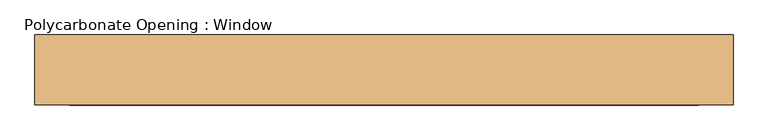
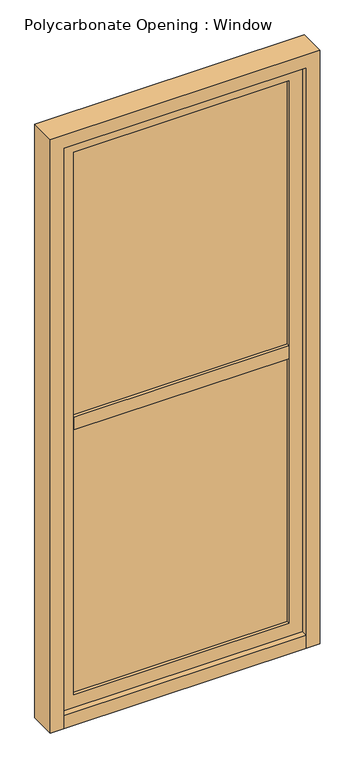
"""IFC4 building model written with IfcOpenShell, lengths in millimetres: door geometry, Polycarbonate Opening : Window."""

from ifc_helpers import new_model, si_unit, frame, origin, origin_with_axes, place, context, project, spatial, polyline, outline, extrude, source, transform, mapped, element, save


def polycarbonate_opening_window_4e587098(model_context):
    return source(origin(), model_context, "Body", "SweptSolid", [
        extrude(outline(polyline([(457.2, 0.0), (457.2, -25.4), (-457.2, -25.4), (-457.2, 0.0), (457.2, 0.0)])), frame((0.0, 0.0, 50.8), z_axis=(0.0, 0.0, 1.0), x_axis=(1.0, 0.0, 0.0)), (0.0, 0.0, 1.0), 2260.6),
        extrude(outline(polyline([(2311.4, -457.2), (0.0, -457.2), (0.0, 457.2), (2311.4, 457.2), (2311.4, -457.2)]), holes=[polyline([(101.6, 406.4), (101.6, -406.4), (2260.6, -406.4), (2260.6, 406.4), (101.6, 406.4)])]), frame((0.0, -38.1, 0.0), z_axis=(0.0, 1.0, 0.0), x_axis=(0.0, 0.0, 1.0)), (0.0, 0.0, 1.0), 50.8),
        extrude(outline(polyline([(2362.2, 508.0), (2362.2, -508.0), (0.0, -508.0), (0.0, -457.2), (2311.4, -457.2), (2311.4, 457.2), (0.0, 457.2), (0.0, 508.0), (2362.2, 508.0)])), frame((0.0, -63.5, 0.0), z_axis=(0.0, 1.0, 0.0), x_axis=(0.0, 0.0, 1.0)), (0.0, 0.0, 1.0), 101.6),
        extrude(outline(polyline([(406.4, 12.7), (406.4, -38.1), (-406.4, -38.1), (-406.4, 12.7), (406.4, 12.7)])), frame((0.0, 0.0, 1155.7), z_axis=(0.0, 0.0, 1.0), x_axis=(1.0, 0.0, 0.0)), (0.0, 0.0, 1.0), 50.8),
        extrude(outline(polyline([(457.2, 38.1), (457.2, -63.5), (-457.2, -63.5), (-457.2, 38.1), (457.2, 38.1)])), origin_with_axes(), (0.0, 0.0, 1.0), 50.8),
    ])


if __name__ == "__main__":
    model = new_model("IFC4")
    model_context = context("Model", 3, world=origin())
    ifc_project = project(units=[si_unit("LENGTHUNIT", "METRE", prefix="MILLI")], contexts=[model_context])
    site = spatial("IfcSite", under=ifc_project)
    building = spatial("IfcBuilding", under=site)
    placement = place(None, origin())
    polycarbonate_opening_window_shape = polycarbonate_opening_window_4e587098(model_context)
    element("IfcDoor", 1, ObjectType="Polycarbonate Opening : Window", at=placement, inside=building, context=model_context, shape_type="MappedRepresentation", body=[
        mapped(polycarbonate_opening_window_shape, transform((0.0, 0.0, 0.0), x_axis=(1.0, 0.0, 0.0), y_axis=(0.0, 1.0, 0.0), z_axis=(0.0, 0.0, 1.0))),
    ])
    save(model, "model.ifc")

# Revit data of these elements
# Type "Polycarbonate Opening : Window"
#   Type Mark = "59"
#   Analytic Construction = "<None>"
#   offset [instance default] = 0' - 2"
#   Stile = 0' - 2"
#   Mullion Width = 0' - 2"
#   Mullion Depth = 0' - 4"
#   Opening Size [instance default] = 5' - 1.50212"
#   Door Width [instance default] = 5' - 1.50212"
#   Window ON/OFF = no
#   Door On/Off = yes
#   Mullion Material = ALUMINUM STOREFRONT
#   Glass Material = INSULATED GLAZING
#   Door Material = ALUMINUM STOREFRONT
# Element 1 (IfcDoor, "Polycarbonate Opening : Window")
#   offset = 0' - 0 1/2"
#   Materials on its faces: "ALUMINUM STOREFRONT", "INSULATED GLAZING"
# Materials
#   "ALUMINUM STOREFRONT": class "Metal", colour RGB 244 244 244, transparency 0, Description = "Aluminum 6061", Cost = 0
#   "INSULATED GLAZING": class "Glass", colour RGB 196 205 210, transparency 0.85, Description = "Soda Lime Glass", Cost = 0
